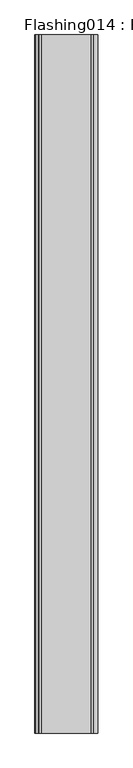
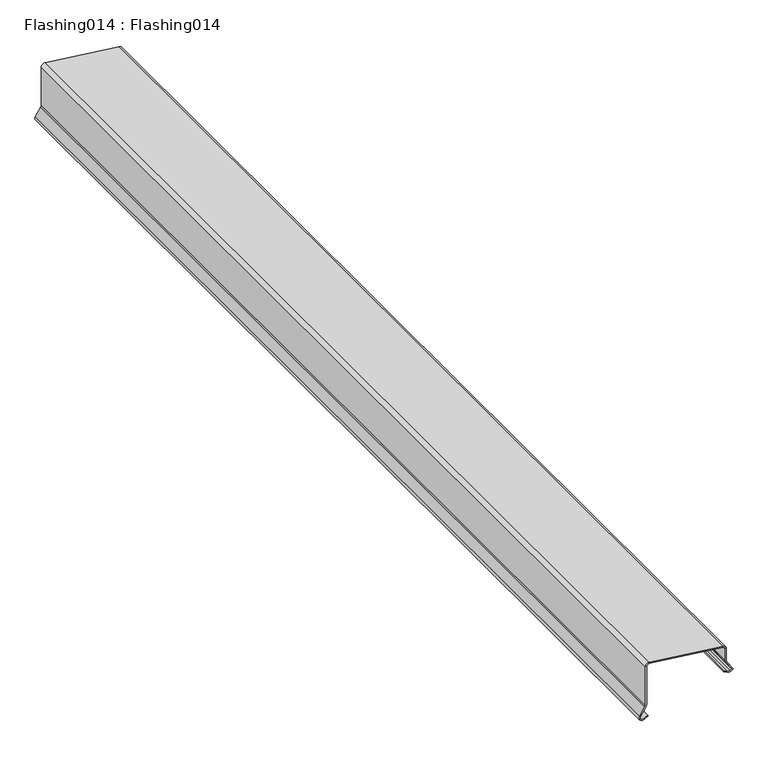
"""IFC4 building model written with IfcOpenShell, lengths in millimetres: proxy geometry, Flashing014 : Flashing014."""

import ifcopenshell
import ifcopenshell.guid

model = None  # the IFC model being written
_history = None  # IfcOwnerHistory: only IFC2X3 demands one
_inside = {}  # id of a spatial element -> (the spatial element, [elements in it])
_under = {}  # id of a project, library or spatial element -> (it, [spatial elements below it])
_declared = {}  # id of a project -> (the project, [libraries it declares])
_typed = {}  # id of a type object -> (the type object, [elements of that type])
_made_of = {}  # id of a material, layer set ... -> (it, [elements and type objects made of it])


def new_model(schema):
    """Start an empty IFC model of exactly this schema.

    Asked for "IFC4X3", IfcOpenShell would pick the latest addendum, in which some entities
    have other attributes; the version numbers below select the first issue.
    IFC2X3 requires an IfcOwnerHistory on every rooted entity: one is made here for all.
    """
    global model, _history
    if schema == "IFC4X3":
        model = ifcopenshell.file(schema_version=(4, 3, 0, 0))
    else:
        model = ifcopenshell.file(schema=schema)
    _inside.clear()
    _under.clear()
    _declared.clear()
    _typed.clear()
    _made_of.clear()
    _history = None
    if model.schema == "IFC2X3":
        org = make("IfcOrganization", Name="unknown")
        user = make(
            "IfcPersonAndOrganization",
            ThePerson=make("IfcPerson", FamilyName="unknown"),
            TheOrganization=org,
        )
        app = make(
            "IfcApplication",
            ApplicationDeveloper=org,
            Version="unknown",
            ApplicationFullName="unknown",
            ApplicationIdentifier="unknown",
        )
        _history = make(
            "IfcOwnerHistory",
            OwningUser=user,
            OwningApplication=app,
            ChangeAction="ADDED",
            CreationDate=0,
        )
    return model


def make(cls, **values):
    """One entity of the class cls with the attributes given. An attribute that is None is left unset."""
    return model.create_entity(
        cls, **{name: value for name, value in values.items() if value is not None}
    )


def rooted(cls, **values):
    """An entity with a GlobalId (a new one), such as an element, a storey or a relation."""
    return make(cls, GlobalId=ifcopenshell.guid.new(), OwnerHistory=_history, **values)


def si_unit(unit_type, name, prefix=None):
    """IfcSIUnit, for example si_unit("LENGTHUNIT", "METRE", prefix="MILLI")."""
    return make("IfcSIUnit", UnitType=unit_type, Prefix=prefix, Name=name)


def assignment(units):
    """IfcUnitAssignment: the units of a project."""
    return None if units is None else make("IfcUnitAssignment", Units=units)


def point(xyz):
    """IfcCartesianPoint."""
    return None if xyz is None else make("IfcCartesianPoint", Coordinates=xyz)


def direction(xyz):
    """IfcDirection."""
    return None if xyz is None else make("IfcDirection", DirectionRatios=xyz)


def frame(location, z_axis=None, x_axis=None):
    """IfcAxis2Placement3D, a coordinate frame: its origin and axes. An axis left out is left unset."""
    return make(
        "IfcAxis2Placement3D",
        Location=point(location),
        Axis=direction(z_axis),
        RefDirection=direction(x_axis),
    )


def frame_2d(location, x_axis=None):
    """IfcAxis2Placement2D, a coordinate frame in the plane: its origin and x axis."""
    return make(
        "IfcAxis2Placement2D", Location=point(location), RefDirection=direction(x_axis)
    )


def origin():
    """The frame at (0, 0, 0) with its axes left unset."""
    return frame((0.0, 0.0, 0.0))


def place(relative_to, where):
    """IfcLocalPlacement: puts the frame where relative to a parent placement (None: the world)."""
    return make(
        "IfcLocalPlacement", PlacementRelTo=relative_to, RelativePlacement=where
    )


def context(
    kind, dimensions, precision=None, world=None, true_north=None, identifier=None
):
    """IfcGeometricRepresentationContext, for example the 3D "Model" context."""
    return make(
        "IfcGeometricRepresentationContext",
        ContextIdentifier=identifier,
        ContextType=kind,
        CoordinateSpaceDimension=dimensions,
        Precision=precision,
        WorldCoordinateSystem=world,
        TrueNorth=true_north,
    )


def project(units=None, contexts=None):
    """IfcProject with its units and contexts."""
    return rooted(
        "IfcProject",
        Name="project",
        RepresentationContexts=contexts,
        UnitsInContext=assignment(units),
    )


def spatial(cls, under=None, at=None, **own):
    """A site, building, storey or space (cls), placed at a placement, below another one or the project."""
    s = rooted(cls, ObjectPlacement=at, **own)
    if under is not None:
        _under.setdefault(under.id(), (under, []))[1].append(s)
    return s


def polyline(points):
    """IfcPolyline through the points."""
    return make("IfcPolyline", Points=[point(p) for p in points])


def circle_curve(where, radius):
    """IfcCircle in the frame where."""
    return make("IfcCircle", Position=where, Radius=radius)


def trimmed(basis, trim1, trim2, sense, master):
    """IfcTrimmedCurve: the piece of a basis curve between two trims."""
    return make(
        "IfcTrimmedCurve",
        BasisCurve=basis,
        Trim1=trim1,
        Trim2=trim2,
        SenseAgreement=sense,
        MasterRepresentation=master,
    )


def segment(curve, same_sense, transition):
    """IfcCompositeCurveSegment."""
    return make(
        "IfcCompositeCurveSegment",
        Transition=transition,
        SameSense=same_sense,
        ParentCurve=curve,
    )


def composite_curve(segments, self_intersect=None):
    """IfcCompositeCurve: segments joined end to end."""
    return make("IfcCompositeCurve", Segments=segments, SelfIntersect=self_intersect)


def outline(outer, holes=None, kind="AREA"):
    """IfcArbitraryClosedProfileDef: a profile drawn as a closed curve; with holes, ...WithVoids."""
    if holes is None:
        return make("IfcArbitraryClosedProfileDef", ProfileType=kind, OuterCurve=outer)
    return make(
        "IfcArbitraryProfileDefWithVoids",
        ProfileType=kind,
        OuterCurve=outer,
        InnerCurves=holes,
    )


def extrude(swept, where, along, depth):
    """IfcExtrudedAreaSolid: the profile swept, set in the frame where, extruded along a direction by depth."""
    return make(
        "IfcExtrudedAreaSolid",
        SweptArea=swept,
        Position=where,
        ExtrudedDirection=direction(along),
        Depth=depth,
    )


def shape(context_of_items, identifier, shape_type, items):
    """IfcShapeRepresentation: the items that make up one representation, for example the "Body"."""
    return make(
        "IfcShapeRepresentation",
        ContextOfItems=context_of_items,
        RepresentationIdentifier=identifier,
        RepresentationType=shape_type,
        Items=items,
    )


def source(mapping_origin, context_of_items, identifier, shape_type, items):
    """IfcRepresentationMap: a shape defined once, which mapped items show again and again."""
    return make(
        "IfcRepresentationMap",
        MappingOrigin=mapping_origin,
        MappedRepresentation=shape(context_of_items, identifier, shape_type, items),
    )


def transform(
    local_origin,
    x_axis=None,
    y_axis=None,
    z_axis=None,
    scale=None,
    scale2=None,
    scale3=None,
    uniform=True,
):
    """IfcCartesianTransformationOperator3D, or its non-uniform kind. x_axis, y_axis, z_axis: its Axis1, 2, 3."""
    if uniform:
        return make(
            "IfcCartesianTransformationOperator3D",
            Axis1=direction(x_axis),
            Axis2=direction(y_axis),
            LocalOrigin=point(local_origin),
            Scale=scale,
            Axis3=direction(z_axis),
        )
    return make(
        "IfcCartesianTransformationOperator3DnonUniform",
        Axis1=direction(x_axis),
        Axis2=direction(y_axis),
        LocalOrigin=point(local_origin),
        Scale=scale,
        Axis3=direction(z_axis),
        Scale2=scale2,
        Scale3=scale3,
    )


def mapped(mapping_source, mapping_target):
    """IfcMappedItem: shows the shape of a source again, moved by a transform."""
    return make(
        "IfcMappedItem", MappingSource=mapping_source, MappingTarget=mapping_target
    )


def made_of(thing, what):
    """Note that an element or type object is made of a material, layer set ...; save() writes the relation."""
    if what is not None:
        _made_of.setdefault(what.id(), (what, []))[1].append(thing)
    return thing


def element(
    cls,
    number,
    at=None,
    inside=None,
    cuts=None,
    type_object=None,
    material=None,
    context=None,
    identifier="Body",
    shape_type=None,
    held_by="IfcProductDefinitionShape",
    body=None,
    shapes=None,
    **own,
):
    """One element of the class cls, such as IfcWall. Its Tag is "e" and its number.

    at: its placement. inside: the storey or other place that contains it. cuts: it is an
    opening in that element (IfcRelVoidsElement). A single representation is given by context,
    identifier, shape_type and body (its items); several are given by shapes. held_by: the class
    of the entity that holds the representations. save() writes the other relations.
    """
    e = rooted(cls, Tag="e%d" % number, ObjectPlacement=at, **own)
    if body is not None:
        shapes = [shape(context, identifier, shape_type, body)]
    if shapes is not None:
        e.Representation = make(held_by, Representations=shapes)
    if inside is not None:
        _inside.setdefault(inside.id(), (inside, []))[1].append(e)
    if cuts is not None:
        rooted(
            "IfcRelVoidsElement", RelatingBuildingElement=cuts, RelatedOpeningElement=e
        )
    if type_object is not None:
        _typed.setdefault(type_object.id(), (type_object, []))[1].append(e)
    return made_of(e, material)


def aggregate(whole, parts):
    """IfcRelAggregates: a whole, such as a stair, and the parts it consists of."""
    return rooted("IfcRelAggregates", RelatingObject=whole, RelatedObjects=parts)


def save(model, path):
    """Write the relations noted so far, then the file.

    IfcRelAggregates (storeys below a building ...), IfcRelContainedInSpatialStructure (elements
    in a storey), IfcRelDefinesByType, IfcRelAssociatesMaterial and IfcRelDeclares: one each for
    every whole, place, type object, material and project.
    """
    for whole, parts in _under.values():
        aggregate(whole, parts)
    for where, things in _inside.values():
        rooted(
            "IfcRelContainedInSpatialStructure",
            RelatedElements=things,
            RelatingStructure=where,
        )
    for kind, things in _typed.values():
        rooted("IfcRelDefinesByType", RelatedObjects=things, RelatingType=kind)
    for what, things in _made_of.values():
        rooted("IfcRelAssociatesMaterial", RelatedObjects=things, RelatingMaterial=what)
    for by, libraries in _declared.values():
        rooted("IfcRelDeclares", RelatingContext=by, RelatedDefinitions=libraries)
    model.write(path)


def flashing014_flashing014_7a834724(model_context):
    return source(origin(), model_context, "Body", "SweptSolid", [
        extrude(outline(composite_curve([segment(trimmed(circle_curve(frame_2d((40133.2517994, -7101.2076081)), 6.35), [point((40127.5360053, -7103.9738687))], [point((40127.867313, -7097.8416304))], False, "CARTESIAN"), True, "CONTINUOUS"), segment(polyline([(40127.867313, -7097.8416304), (40130.8867187, -7093.0115482), (40149.4789842, -7105.0053963)]), True, "CONTINUOUS"), segment(trimmed(circle_curve(frame_2d((40152.9212544, -7099.6693607)), 6.35), [point((40149.4789842, -7105.0053963))], [point((40152.9212544, -7106.0193607))], True, "CARTESIAN"), True, "CONTINUOUS"), segment(polyline([(40152.9212544, -7106.0193607), (40176.1640916, -7106.0193607)]), True, "CONTINUOUS"), segment(trimmed(circle_curve(frame_2d((40176.1640916, -7112.3693607)), 6.35), [point((40176.1640916, -7106.0193607))], [point((40182.4677067, -7111.6032428))], False, "CARTESIAN"), True, "CONTINUOUS"), segment(polyline([(40182.4677067, -7111.6032428), (40199.6976336, -7253.3710163)]), True, "CONTINUOUS"), segment(trimmed(circle_curve(frame_2d((40193.3940184, -7254.1371341)), 6.35), [point((40199.6976336, -7253.3710163))], [point((40193.3940184, -7260.4871341))], False, "CARTESIAN"), True, "CONTINUOUS"), segment(polyline([(40193.3940184, -7260.4871341), (40116.1659228, -7260.4871341)]), True, "CONTINUOUS"), segment(trimmed(circle_curve(frame_2d((40116.1659228, -7266.8371341)), 6.35), [point((40116.1659228, -7260.4871341))], [point((40112.7319037, -7261.4957849))], True, "CARTESIAN"), True, "CONTINUOUS"), segment(polyline([(40112.7319037, -7261.4957849), (40096.8914441, -7271.6798112)]), True, "CONTINUOUS"), segment(trimmed(circle_curve(frame_2d((40093.4574249, -7266.3384619)), 6.35), [point((40096.8914441, -7271.6798112))], [point((40088.1090015, -7269.7614529))], False, "CARTESIAN"), True, "CONTINUOUS"), segment(polyline([(40088.1090015, -7269.7614529), (40086.3359375, -7266.9910404), (40092.1875, -7255.2840091), (40093.9764738, -7256.1781976), (40088.63264, -7266.8694325), (40089.7935443, -7268.6833455)]), True, "CONTINUOUS"), segment(trimmed(circle_curve(frame_2d((40093.4574249, -7266.3384619)), 4.35), [point((40089.7935443, -7268.6833455))], [point((40095.8098632, -7269.9974965))], True, "CARTESIAN"), True, "CONTINUOUS"), segment(polyline([(40095.8098632, -7269.9974965), (40111.6503228, -7259.8134701)]), True, "CONTINUOUS"), segment(trimmed(circle_curve(frame_2d((40116.1659228, -7266.8371341)), 8.35), [point((40111.6503228, -7259.8134701))], [point((40116.1659228, -7258.4871341))], False, "CARTESIAN"), True, "CONTINUOUS"), segment(polyline([(40116.1659228, -7258.4871341), (40193.3940184, -7258.4871341)]), True, "CONTINUOUS"), segment(trimmed(circle_curve(frame_2d((40193.3940184, -7254.1371341)), 4.35), [point((40193.3940184, -7258.4871341))], [point((40197.712243, -7253.6123132))], True, "CARTESIAN"), True, "CONTINUOUS"), segment(polyline([(40197.712243, -7253.6123132), (40180.4823161, -7111.8445398)]), True, "CONTINUOUS"), segment(trimmed(circle_curve(frame_2d((40176.1640916, -7112.3693607)), 4.35), [point((40180.4823161, -7111.8445398))], [point((40176.1640916, -7108.0193607))], True, "CARTESIAN"), True, "CONTINUOUS"), segment(polyline([(40176.1640916, -7108.0193607), (40152.9212544, -7108.0193607)]), True, "CONTINUOUS"), segment(trimmed(circle_curve(frame_2d((40152.9212544, -7099.6693607)), 8.35), [point((40152.9212544, -7108.0193607))], [point((40148.3948046, -7106.6860375))], False, "CARTESIAN"), True, "CONTINUOUS"), segment(polyline([(40148.3948046, -7106.6860375), (40131.5072723, -7095.7919106), (40129.5632143, -7098.9017809)]), True, "CONTINUOUS"), segment(trimmed(circle_curve(frame_2d((40133.2517994, -7101.2076081)), 4.35), [point((40129.5632143, -7098.9017809))], [point((40129.3362554, -7103.1026055))], True, "CARTESIAN"), True, "CONTINUOUS"), segment(polyline([(40129.3362554, -7103.1026055), (40132.6869689, -7110.0260272), (40130.8867187, -7110.8972904), (40127.5360053, -7103.9738687)]), True, "CONTINUOUS")], self_intersect=False)), frame((0.0, 7982.1531721, 0.0), z_axis=(0.0, 1.0, 0.0), x_axis=(0.0, 0.0, 1.0)), (0.0, 0.0, 1.0), 2000.0),
    ])


if __name__ == "__main__":
    model = new_model("IFC4")
    model_context = context("Model", 3, world=origin())
    ifc_project = project(units=[si_unit("LENGTHUNIT", "METRE", prefix="MILLI")], contexts=[model_context])
    site = spatial("IfcSite", under=ifc_project)
    building = spatial("IfcBuilding", under=site)
    placement = place(None, origin())
    flashing014_flashing014_shape = flashing014_flashing014_7a834724(model_context)
    element("IfcBuildingElementProxy", 1, Name="Flashing014 : Flashing014", ObjectType="Flashing014 : Flashing014", at=placement, inside=building, context=model_context, shape_type="MappedRepresentation", body=[
        mapped(flashing014_flashing014_shape, transform((0.0, 0.0, 0.0), x_axis=(1.0, 0.0, 0.0), y_axis=(0.0, 1.0, 0.0), z_axis=(0.0, 0.0, 1.0))),
    ])
    save(model, "model.ifc")

# Revit data of these elements
# Type "Flashing014 : Flashing014"
#   NameOverride = "Flashing014"
# Element 1 (IfcBuildingElementProxy, "Flashing014 : Flashing014")
#   Materials on its faces: "METAL COPING"
# Materials
#   "METAL COPING": class "Unassigned", colour RGB 128 128 128, transparency 0
